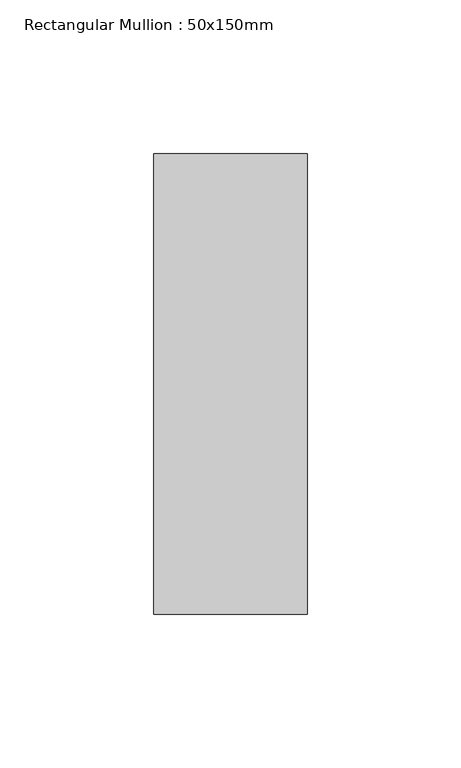
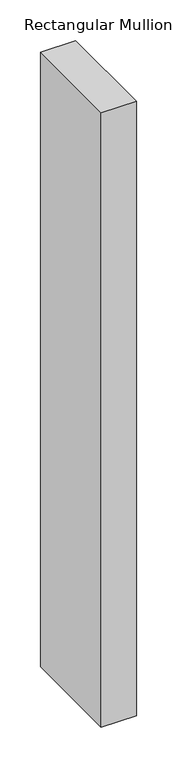
"""IFC4 building model written with IfcOpenShell, lengths in millimetres: member geometry, Rectangular Mullion : 50x150mm."""

from ifc_helpers import new_model, si_unit, frame, origin, place, context, project, spatial, polyline, outline, extrude, source, transform, mapped, element, save


def rectangular_mullion_50x150mm_a91aaa2b(model_context):
    return source(origin(), model_context, "Body", "SweptSolid", [
        extrude(outline(polyline([(0.0, 75.0), (0.0, -75.0), (-50.0, -75.0), (-50.0, 75.0), (0.0, 75.0)])), frame((0.0, 0.0, -925.0), z_axis=(0.0, 0.0, 1.0), x_axis=(1.0, 0.0, 0.0)), (0.0, 0.0, 1.0), 925.0),
    ])


if __name__ == "__main__":
    model = new_model("IFC4")
    model_context = context("Model", 3, world=origin())
    ifc_project = project(units=[si_unit("LENGTHUNIT", "METRE", prefix="MILLI")], contexts=[model_context])
    site = spatial("IfcSite", under=ifc_project)
    building = spatial("IfcBuilding", under=site)
    placement = place(None, origin())
    rectangular_mullion_50x150mm_shape = rectangular_mullion_50x150mm_a91aaa2b(model_context)
    element("IfcMember", 1, ObjectType="Rectangular Mullion : 50x150mm", at=placement, inside=building, context=model_context, shape_type="MappedRepresentation", body=[
        mapped(rectangular_mullion_50x150mm_shape, transform((0.0, 0.0, 0.0), x_axis=(1.0, 0.0, 0.0), y_axis=(0.0, 1.0, 0.0), z_axis=(0.0, 0.0, 1.0))),
    ])
    save(model, "model.ifc")

# Revit data of these elements
# Type "Rectangular Mullion : 50x150mm"
#   Keynote = "H11"
#   built-in parameter 1007304 = 0.492126 (stored number, unit not read)
#   built-in parameter 1007301 = 0.082021 (stored number, unit not read)
#   built-in parameter 1007300 = 0.082021 (stored number, unit not read)
# Element 1 (IfcMember, "Rectangular Mullion : 50x150mm")
#   Materials on its faces: "Aluminium"
# Materials
#   "Aluminium": class "Metal", colour RGB 247 247 247, transparency 0, Description = "Aluminium 6061", Cost = 0
